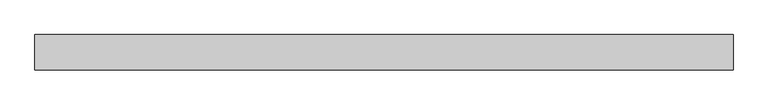
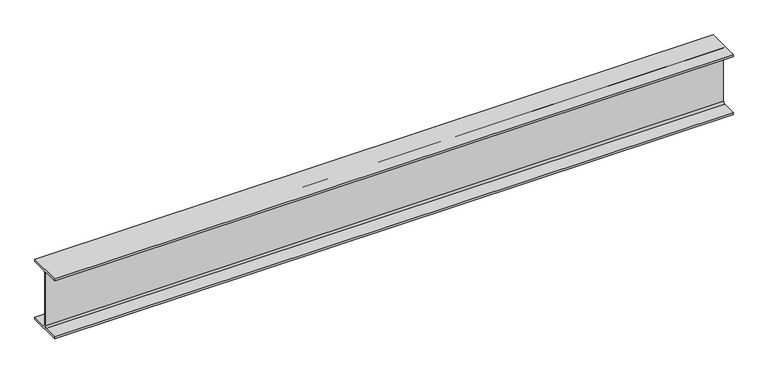
"""IFC4 building model written with IfcOpenShell, lengths in millimetres: beam geometry, Old_Steel Beam_H-KSD3502 : H_SB_ASB_H-200×200x8x12."""

from ifc_helpers import new_model, si_unit, point, frame, frame_2d, origin, place, context, project, spatial, polyline, circle_curve, trimmed, segment, composite_curve, outline, extrude, source, transform, mapped, element, save


def beam_f9cf12d6(model_context):
    return source(origin(), model_context, "Body", "SweptSolid", [
        extrude(outline(composite_curve([segment(polyline([(82.5, -141.5), (82.5, -151.7), (-82.5, -151.7), (-82.5, -141.5), (-11.9, -141.5)]), True, "CONTINUOUS"), segment(trimmed(circle_curve(frame_2d((-11.9, -132.6)), 8.9), [point((-11.9, -141.5))], [point((-3.0, -132.6))], True, "CARTESIAN"), True, "CONTINUOUS"), segment(polyline([(-3.0, -132.6), (-3.0, 132.6)]), True, "CONTINUOUS"), segment(trimmed(circle_curve(frame_2d((-11.9, 132.6)), 8.9), [point((-3.0, 132.6))], [point((-11.9, 141.5))], True, "CARTESIAN"), True, "CONTINUOUS"), segment(polyline([(-11.9, 141.5), (-82.5, 141.5), (-82.5, 151.7), (82.5, 151.7), (82.5, 141.5), (11.9, 141.5)]), True, "CONTINUOUS"), segment(trimmed(circle_curve(frame_2d((11.9, 132.6)), 8.9), [point((11.9, 141.5))], [point((3.0, 132.6))], True, "CARTESIAN"), True, "CONTINUOUS"), segment(polyline([(3.0, 132.6), (3.0, -132.6)]), True, "CONTINUOUS"), segment(trimmed(circle_curve(frame_2d((11.9, -132.6)), 8.9), [point((3.0, -132.6))], [point((11.9, -141.5))], True, "CARTESIAN"), True, "CONTINUOUS"), segment(polyline([(11.9, -141.5), (82.5, -141.5)]), True, "CONTINUOUS")], self_intersect=False)), frame((-1415.8166437, 0.0, 0.0), z_axis=(1.0, 0.0, 0.0), x_axis=(0.0, 1.0, 0.0)), (0.0, 0.0, 1.0), 3239.5063623),
    ])


if __name__ == "__main__":
    model = new_model("IFC4")
    model_context = context("Model", 3, world=origin())
    ifc_project = project(units=[si_unit("LENGTHUNIT", "METRE", prefix="MILLI")], contexts=[model_context])
    site = spatial("IfcSite", under=ifc_project)
    building = spatial("IfcBuilding", under=site)
    placement = place(None, origin())
    beam_shape = beam_f9cf12d6(model_context)
    element("IfcBeam", 1, ObjectType="Old_Steel Beam_H-KSD3502 : H_SB_ASB_H-200×200x8x12", at=placement, inside=building, context=model_context, shape_type="MappedRepresentation", body=[
        mapped(beam_shape, transform((0.0, 0.0, 0.0), x_axis=(1.0, 0.0, 0.0), y_axis=(0.0, 1.0, 0.0), z_axis=(0.0, 0.0, 1.0))),
    ])
    save(model, "model.ifc")

# Revit data of these elements
# Type "Old_Steel Beam_H-KSD3502 : H_SB_ASB_H-200×200x8x12"
#   Width = 20.0 cm
#   Web Thickness = 0.8 cm
#   Web Fillet = 1.3 cm
#   Warping Constant = 141376.0 cm⁶
#   Torsional Moment of Inertia = 26.2485 cm⁴
#   Torsional Modulus = 1.0 cm³
#   Section Area = 63.53 cm²
#   Plastic Modulus weak axis = 244.0 cm³
#   Plastic Modulus strong axis = 525.0 cm³
#   Perimeter = 1.16 m²/m
#   Nominal Weight = 49.90 kgf/m
#   Moment of Inertia weak axis = 1600.00 cm⁴
#   Moment of Inertia strong axis = 4720.00 cm⁴
#   Height = 20.0 cm
#   Flange Thickness = 1.2 cm
#   Elastic Modulus weak axis = 160.0 cm³
#   Elastic Modulus strong axis = 472.0 cm³
#   Centroid Vertical = 10.0 cm
#   Centroid Horizontal = 10.0 cm
#   Length [instance default] = 1.5240 m
#   Structural Material [instance default] = Steel, 45-345
#   Assembly Code = ""
# Element 1 (IfcBeam, "Old_Steel Beam_H-KSD3502 : H_SB_ASB_H-200×200x8x12")
#   Structural Material = none
# Materials
#   "Steel, 45-345": class "Metal", colour RGB 189 187 185, transparency 0, Description = "Steel 345 MPa", Cost = 0
